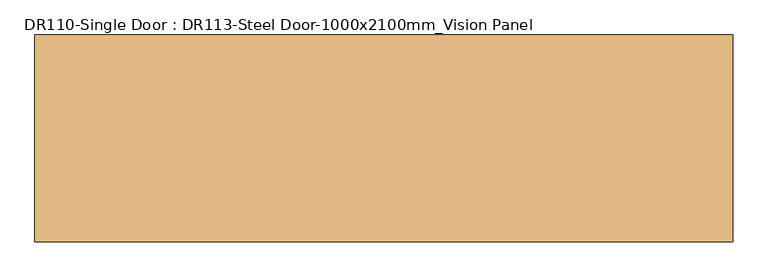
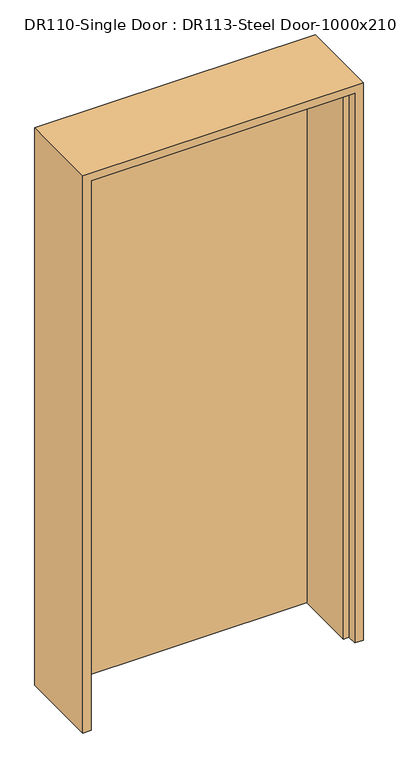
"""IFC4 building model written with IfcOpenShell, lengths in millimetres: door geometry, DR110-Single Door : DR113-Steel Door-1000x2100mm_Vision Panel."""

from ifc_helpers import new_model, si_unit, origin, origin_with_axes, place, context, project, spatial, polyline, outline, extrude, faceted_brep, source, transform, mapped, element, save


def dr110_single_door_dr113_steel_door_1000x2100mm_vision_panel_a59affbd(model_context):
    return source(origin(), model_context, "Body", "SolidModel", [
        extrude(outline(polyline([(470.0, 148.0), (470.0, 113.0), (-470.0, 113.0), (-470.0, 148.0), (470.0, 148.0)])), origin_with_axes(), (0.0, 0.0, 1.0), 2070.0),
        faceted_brep([(470.0, 148.0, 0.0), (500.0, 148.0, 0.0), (500.0, -148.0, 0.0), (470.0, -148.0, 0.0), (470.0, -113.0, 0.0), (450.0, -113.0, 0.0), (450.0, 113.0, 0.0), (470.0, 113.0, 0.0), (470.0, 148.0, 2070.0), (-470.0, 148.0, 2070.0), (-470.0, 148.0, 0.0), (-500.0, 148.0, 0.0), (-500.0, 148.0, 2100.0), (500.0, 148.0, 2100.0), (500.0, -148.0, 2100.0), (-500.0, -148.0, 2100.0), (-500.0, -148.0, 0.0), (-470.0, -148.0, 0.0), (-470.0, -148.0, 2070.0), (470.0, -148.0, 2070.0), (470.0, -113.0, 2070.0), (-470.0, -113.0, 2070.0), (-470.0, -113.0, 0.0), (-450.0, -113.0, 0.0), (-450.0, -113.0, 2050.0), (450.0, -113.0, 2050.0), (450.0, 113.0, 2050.0), (-450.0, 113.0, 2050.0), (-450.0, 113.0, 0.0), (-470.0, 113.0, 0.0), (-470.0, 113.0, 2070.0), (470.0, 113.0, 2070.0)], [[[0, 1, 2, 3, 4, 5, 6, 7]], [[1, 0, 8, 9, 10, 11, 12, 13]], [[2, 1, 13, 14]], [[3, 2, 14, 15, 16, 17, 18, 19]], [[4, 3, 19, 20]], [[5, 4, 20, 21, 22, 23, 24, 25]], [[6, 5, 25, 26]], [[7, 6, 26, 27, 28, 29, 30, 31]], [[0, 7, 31, 8]], [[9, 30, 29, 10]], [[10, 29, 28, 23, 22, 17, 16, 11]], [[15, 12, 11, 16]], [[21, 18, 17, 22]], [[27, 24, 23, 28]], [[14, 13, 12, 15]], [[20, 19, 18, 21]], [[26, 25, 24, 27]], [[8, 31, 30, 9]]]),
    ])


if __name__ == "__main__":
    model = new_model("IFC4")
    model_context = context("Model", 3, world=origin())
    ifc_project = project(units=[si_unit("LENGTHUNIT", "METRE", prefix="MILLI")], contexts=[model_context])
    site = spatial("IfcSite", under=ifc_project)
    building = spatial("IfcBuilding", under=site)
    placement = place(None, origin())
    dr110_single_door_dr113_steel_door_1000x2100mm_vision_panel_shape = dr110_single_door_dr113_steel_door_1000x2100mm_vision_panel_a59affbd(model_context)
    element("IfcDoor", 1, ObjectType="DR110-Single Door : DR113-Steel Door-1000x2100mm_Vision Panel", at=placement, inside=building, context=model_context, shape_type="MappedRepresentation", body=[
        mapped(dr110_single_door_dr113_steel_door_1000x2100mm_vision_panel_shape, transform((0.0, 0.0, 0.0), x_axis=(1.0, 0.0, 0.0), y_axis=(0.0, 1.0, 0.0), z_axis=(0.0, 0.0, 1.0))),
    ])
    save(model, "model.ifc")

# Revit data of these elements
# Type "DR110-Single Door : DR113-Steel Door-1000x2100mm_Vision Panel"
#   Type Mark = "SD"
#   Analytic Construction = "<None>"
#   프레임 투영 외부. = 25 mm
#   프레임 투영 내부. = 25 mm
#   프레임 폭 = 75 mm
#   Height = 2100 mm
#   Width = 1000 mm
#   Define Thermal Properties by = 1
#   문 패널 = SD1 문 패널
#   문 프레임 = A04AQ098-00002_Steel Door_non FP_single
#   Function = (empty or 0)
#   Wall Closure = (empty or 0)
# Element 1 (IfcDoor, "DR110-Single Door : DR113-Steel Door-1000x2100mm_Vision Panel")
#   Materials on its faces: "A04AQ098-00002_Steel Door_non FP_single", "SD1 문 패널"
# Materials
#   "SD1 문 패널": class "금속", colour RGB 247 247 247, transparency 0, Description = "STEEL DOOR (1000Wx2100H)"
#   "A04AQ098-00002_Steel Door_non FP_single": class "금속", colour RGB 247 247 247, transparency 0, Description = "Steel Door", W00) Work Master Code = "A04AQ098-00002", W01) Work Master_Lv1 = "Finishing Work", W02) Work Master_Lv2 = "Door & Window Work", W03) Work Master_Spec.1 = "Steel Door w/ Steel Frame", W04) Work Master_Spec.2 = "Fire Protective Rating: N/A, Single Door", W05) Work Master_Spec.3 = "w/ Hardware & Accessories", Cost = 0
